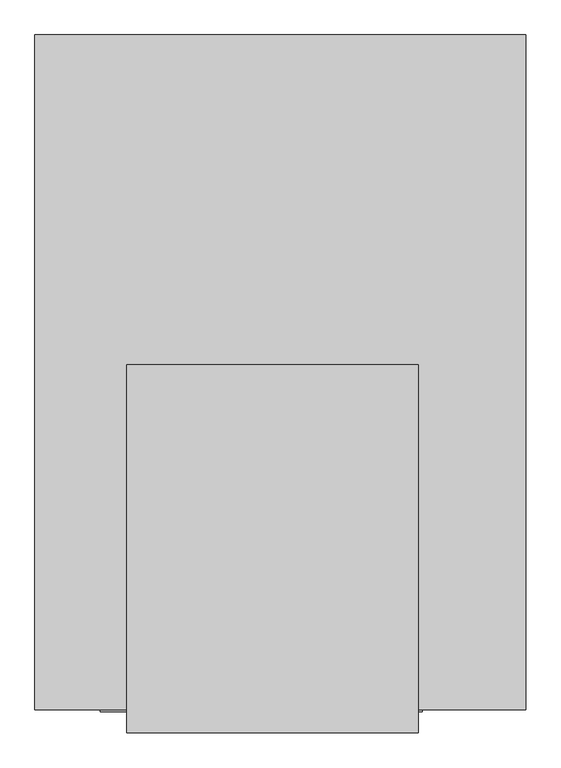
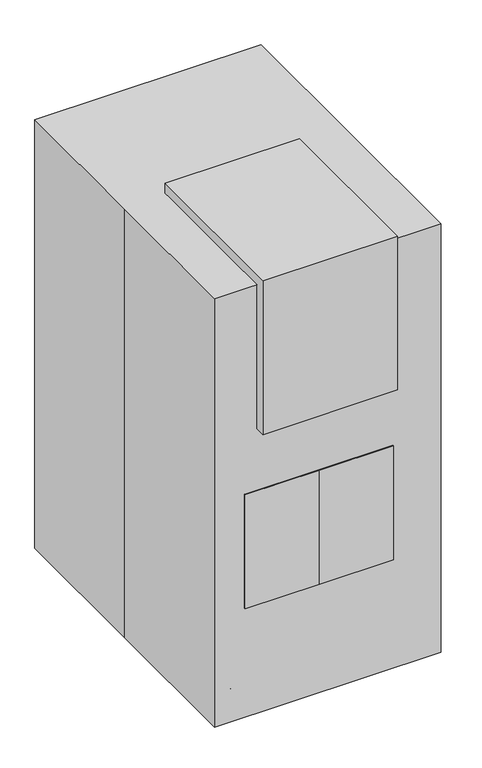
"""IFC4 building model written with IfcOpenShell, lengths in millimetres: proxy geometry, X9500 - System, Uptake, Thyroid, Mobile : X9500 - System, Uptake, Thyroid, Mobile."""

from ifc_helpers import new_model, si_unit, point, frame, frame_2d, origin, origin_with_axes, place, context, project, spatial, polyline, circle_curve, trimmed, segment, composite_curve, outline, extrude, faceted_brep, source, transform, mapped, element, save


def specialty_equipment_a1d769d3(model_context):
    return source(origin(), model_context, "Body", "SolidModel", [
        faceted_brep([(222.25, -92.075, 768.5274151), (-208.9546875, -92.075, 768.5274151), (-208.9546875, -307.975, 768.5274151), (222.25, -307.975, 768.5274151), (222.25, -523.875, 412.9274151), (-208.9546875, -523.875, 412.9274151), (-208.9546875, -92.075, 412.9274151), (222.25, -92.075, 412.9274151), (222.25, -307.975, 735.7348675), (222.25, -523.875, 735.7348675), (222.25, -523.875, 590.7274151), (222.25, -307.975, 590.7274151), (222.25, -307.975, 495.1924677), (222.25, -523.875, 533.6276131), (-208.9546875, -523.875, 533.6276131), (163.7431114, -523.875, 735.7348675), (163.7431114, -523.875, 666.9274151), (-161.3296875, -523.875, 666.9274151), (-161.3296875, -523.875, 735.7348675), (-208.9546875, -523.875, 735.7348675), (-208.9546875, -523.875, 666.9274151), (-285.75, -523.875, 666.9274151), (-285.75, -523.875, 590.7274151), (-285.75, -92.075, 666.9274151), (-285.75, -92.075, 590.7274151), (-208.9546875, -92.075, 590.7274151), (-208.9546875, -92.075, 666.9274151), (163.7431114, -307.975, 735.7348675), (-161.3296875, -307.975, 735.7348675), (-208.9546875, -307.975, 735.7348675), (-161.3296875, -307.975, 666.9274151), (163.7431114, -307.975, 666.9274151), (-208.9546875, -307.975, 590.7274151), (-208.9546875, -307.975, 495.1924677)], [[[0, 1, 2, 3]], [[4, 5, 6, 7]], [[7, 0, 3, 8, 9, 10, 11, 12, 13, 4]], [[13, 14, 5, 4]], [[15, 16, 17, 18, 19, 20, 21, 22, 10, 9]], [[23, 24, 22, 21]], [[7, 6, 25, 24, 23, 26, 1, 0]], [[8, 27, 15, 9]], [[28, 29, 19, 18]], [[3, 2, 29, 28, 30, 31, 27, 8]], [[30, 28, 18, 17]], [[30, 17, 16, 31]], [[16, 15, 27, 31]], [[26, 23, 21, 20]], [[20, 19, 29, 2, 1, 26]], [[10, 22, 24, 25, 32, 11]], [[12, 33, 14, 13]], [[11, 32, 33, 12]], [[25, 6, 5, 14, 33, 32]]]),
        extrude(outline(polyline([(234.95, -561.975), (-31.75, -561.975), (-298.45, -561.975), (-298.45, -53.975), (234.95, -53.975), (234.95, -561.975)])), frame((0.0, 0.0, 412.9274151), z_axis=(0.0, 0.0, 1.0), x_axis=(1.0, 0.0, 0.0)), (0.0, 0.0, 1.0), 431.8),
        faceted_brep([(-145.9656905, -533.4, 1511.3), (-95.3343095, -533.4, 1511.3), (-95.3343095, -50.8, 1511.3), (-145.9656905, -50.8, 1511.3), (-145.9656905, -533.4, 1231.9), (-145.9656905, -50.8, 1231.9), (-95.3343095, -50.8, 1231.9), (-95.3343095, -533.4, 1231.9), (-95.3343095, -63.5, 1498.6), (-95.3343095, -63.5, 1244.6), (-95.3343095, -520.7, 1244.6), (-95.3343095, -520.7, 1498.6), (-100.1205119, -520.7, 1498.6), (-100.1205119, -63.5, 1498.6), (-100.1205119, -520.7, 1244.6), (-100.1205119, -63.5, 1244.6)], [[[0, 1, 2, 3]], [[4, 5, 6, 7]], [[3, 5, 4, 0]], [[2, 6, 5, 3]], [[1, 7, 6, 2], [8, 9, 10, 11]], [[0, 4, 7, 1]], [[12, 13, 8, 11]], [[14, 10, 9, 15]], [[12, 14, 15, 13]], [[13, 15, 9, 8]], [[11, 10, 14, 12]]]),
        extrude(outline(polyline([(1092.2, 203.2), (1104.9, 50.8), (1079.5, 50.8), (1079.5, 203.2), (1092.2, 203.2)])), frame((0.0, -533.4, 0.0), z_axis=(0.0, 1.0, 0.0), x_axis=(0.0, 0.0, 1.0)), (0.0, 0.0, 1.0), 482.6),
        faceted_brep([(-12.7, -439.3218395, 1104.9), (-228.6, -439.3218395, 1104.9), (-228.6, -439.3218395, 1079.5), (-12.7, -439.3218395, 1079.5), (-228.6, -144.8781605, 1104.9), (-12.7, -144.8781605, 1104.9), (-12.7, -144.8781605, 1079.5), (-228.6, -144.8781605, 1079.5), (-209.4656905, -329.0685686, 1111.25), (-209.4656905, -255.1314314, 1111.25), (-209.4656905, -255.1314314, 1104.9), (-209.4656905, -329.0685686, 1104.9), (-209.4656905, -329.0685686, 1371.6), (-209.4656905, -255.1314314, 1371.6), (-145.9656905, -329.0685686, 1371.6), (-145.9656905, -255.1314314, 1371.6), (-145.9656905, -329.0685686, 1320.8), (-145.9656905, -255.1314314, 1320.8), (-184.0656905, -329.0685686, 1320.8), (-184.0656905, -255.1314314, 1320.8), (-184.0656905, -329.0685686, 1104.9), (-184.0656905, -255.1314314, 1104.9)], [[[0, 1, 2, 3]], [[4, 5, 6, 7]], [[8, 9, 10, 11]], [[12, 13, 9, 8]], [[14, 15, 13, 12]], [[16, 17, 15, 14]], [[18, 19, 17, 16]], [[20, 21, 19, 18]], [[0, 5, 4, 1], [11, 10, 21, 20]], [[3, 6, 5, 0]], [[2, 7, 6, 3]], [[1, 4, 7, 2]], [[20, 18, 16, 14, 12, 8, 11]], [[10, 9, 13, 15, 17, 19, 21]]]),
        extrude(outline(polyline([(-254.0, -596.9), (-254.0, 12.7), (228.6, 12.7), (228.6, -596.9), (-254.0, -596.9)])), frame((0.0, 0.0, 1079.5), z_axis=(0.0, 0.0, 1.0), x_axis=(1.0, 0.0, 0.0)), (0.0, 0.0, 1.0), 584.2),
        extrude(outline(composite_curve([segment(polyline([(119.1380154, 235.2310593), (119.1380154, 381.2810593), (123.8052853, 381.2810593), (123.8052853, 235.359733)]), True, "CONTINUOUS"), segment(trimmed(circle_curve(frame_2d((11.7763715, 229.2430177)), 112.1957741), [point((123.8052853, 235.359733))], [point((77.7346619, 138.4829182))], False, "CARTESIAN"), True, "CONTINUOUS"), segment(polyline([(77.7346619, 138.4829182), (-77.7346619, 138.4829182)]), True, "CONTINUOUS"), segment(trimmed(circle_curve(frame_2d((-11.7763715, 229.2430177)), 112.1957741), [point((-77.7346619, 138.4829182))], [point((-123.8052853, 235.359733))], False, "CARTESIAN"), True, "CONTINUOUS"), segment(polyline([(-123.8052853, 235.359733), (-123.8052853, 381.2810593), (-119.1380154, 381.2810593), (-119.1380154, 235.2310593)]), True, "CONTINUOUS"), segment(trimmed(circle_curve(frame_2d((-11.7763715, 229.2430177)), 107.5285042), [point((-119.1380154, 235.2310593))], [point((-76.2, 143.1501881))], True, "CARTESIAN"), True, "CONTINUOUS"), segment(polyline([(-76.2, 143.1501881), (76.2, 143.1501881)]), True, "CONTINUOUS"), segment(trimmed(circle_curve(frame_2d((11.7763715, 229.2430177)), 107.5285042), [point((76.2, 143.1501881))], [point((119.1380154, 235.2310593))], True, "CARTESIAN"), True, "CONTINUOUS")], self_intersect=False)), frame((0.0, 0.0, 1016.0), z_axis=(0.0, 0.0, 1.0), x_axis=(1.0, 0.0, 0.0)), (0.0, 0.0, 1.0), 19.05),
        extrude(outline(polyline([(0.0, 271.5253368), (238.2760308, 271.5253368), (238.2760308, 0.0), (0.0, 0.0), (0.0, 271.5253368)])), frame((119.1380154, 525.6105842, 1054.6277039), z_axis=(0.0, -0.3583679495452942, 0.9335804264972041), x_axis=(-1.0, 0.0, 0.0)), (0.0, 0.0, 1.0), 50.8),
        extrude(outline(polyline([(50.8, 36.8829182), (-50.8, 36.8829182), (-50.8, 138.4829182), (50.8, 138.4829182), (50.8, 36.8829182)])), frame((0.0, 0.0, 1004.2876576), z_axis=(0.0, 0.0, 1.0), x_axis=(1.0, 0.0, 0.0)), (0.0, 0.0, 1.0), 50.8),
        extrude(outline(polyline([(203.2, -547.3170818), (-209.55, -547.3170818), (-209.55, -39.3170818), (203.2, -39.3170818), (203.2, -547.3170818)])), frame((0.0, 0.0, 374.65), z_axis=(0.0, 0.0, 1.0), x_axis=(1.0, 0.0, 0.0)), (0.0, 0.0, 1.0), 38.1),
        extrude(outline(polyline([(-39.3170818, 1041.4), (-39.3170818, 812.8), (-191.7170818, 812.8), (-521.9170818, 1016.0), (-521.9170818, 1041.4), (-39.3170818, 1041.4)])), frame((190.5, 0.0, 0.0), z_axis=(1.0, 0.0, 0.0), x_axis=(0.0, 1.0, 0.0)), (0.0, 0.0, 1.0), 38.1),
        extrude(outline(polyline([(-39.3170818, 1041.4), (-39.3170818, 812.8), (-191.7170818, 812.8), (-521.9170818, 1016.0), (-521.9170818, 1041.4), (-39.3170818, 1041.4)])), frame((-228.6, 0.0, 0.0), z_axis=(1.0, 0.0, 0.0), x_axis=(0.0, 1.0, 0.0)), (0.0, 0.0, 1.0), 38.1),
        extrude(outline(polyline([(247.65, -547.3170818), (-253.5329849, -547.3170818), (-253.5329849, -39.3170818), (247.65, -39.3170818), (247.65, -547.3170818)])), frame((0.0, 0.0, 1041.4), z_axis=(0.0, 0.0, 1.0), x_axis=(1.0, 0.0, 0.0)), (0.0, 0.0, 1.0), 38.1),
        extrude(outline(polyline([(-209.55, -39.3170818), (-209.55, -83.7670818), (-304.8, -83.7670818), (-304.8, 83.7670818), (-209.55, 83.7670818), (-209.55, 36.8829182), (-254.0, 36.8829182), (-254.0, -1.2170818), (-254.0, -39.3170818), (-209.55, -39.3170818)])), frame((0.0, 0.0, 266.7), z_axis=(0.0, 0.0, 1.0), x_axis=(1.0, 0.0, 0.0)), (0.0, 0.0, 1.0), 342.9),
        extrude(outline(polyline([(203.2, -39.3170818), (247.65, -39.3170818), (247.65, -1.2170818), (247.65, 36.8829182), (203.2, 36.8829182), (203.2, 83.7670818), (298.45, 83.7670818), (298.45, -83.7670818), (203.2, -83.7670818), (203.2, -39.3170818)])), frame((0.0, 0.0, 266.7), z_axis=(0.0, 0.0, 1.0), x_axis=(1.0, 0.0, 0.0)), (0.0, 0.0, 1.0), 342.9),
        extrude(outline(polyline([(247.65, -39.3170818), (-253.5329849, -39.3170818), (-253.5329849, 36.8829182), (247.65, 36.8829182), (247.65, -39.3170818)])), frame((0.0, 0.0, 266.7), z_axis=(0.0, 0.0, 1.0), x_axis=(1.0, 0.0, 0.0)), (0.0, 0.0, 1.0), 1248.8024583),
        extrude(outline(polyline([(349.25, -121.8929078), (-355.1329849, -121.8929078), (-355.1329849, 133.5826903), (349.25, 133.5826903), (349.25, -121.8929078)])), frame((0.0, 0.0, 165.1), z_axis=(0.0, 0.0, 1.0), x_axis=(1.0, 0.0, 0.0)), (0.0, 0.0, 1.0), 101.6),
        extrude(outline(composite_curve([segment(trimmed(circle_curve(frame_2d((-306.4724956, 409.1524744)), 16.9333333), [point((-323.405829, 409.1524744))], [point((-289.5391623, 409.1524744))], False, "CARTESIAN"), True, "CONTINUOUS"), segment(trimmed(circle_curve(frame_2d((-306.4724956, 409.1524744)), 16.9333333), [point((-289.5391623, 409.1524744))], [point((-323.405829, 409.1524744))], False, "CARTESIAN"), True, "CONTINUOUS")], self_intersect=False)), frame((0.0, 0.0, 84.8149176), z_axis=(0.0, 0.0, 1.0), x_axis=(1.0, 0.0, 0.0)), (0.0, 0.0, 1.0), 42.1850824),
        extrude(outline(composite_curve([segment(trimmed(circle_curve(frame_2d((297.8141923, 409.1524744)), 16.9333333), [point((314.7475256, 409.1524744))], [point((280.880859, 409.1524744))], False, "CARTESIAN"), True, "CONTINUOUS"), segment(trimmed(circle_curve(frame_2d((297.8141923, 409.1524744)), 16.9333333), [point((280.880859, 409.1524744))], [point((314.7475256, 409.1524744))], False, "CARTESIAN"), True, "CONTINUOUS")], self_intersect=False)), frame((0.0, 0.0, 84.8149176), z_axis=(0.0, 0.0, 1.0), x_axis=(1.0, 0.0, 0.0)), (0.0, 0.0, 1.0), 42.1850824),
        extrude(outline(composite_curve([segment(trimmed(circle_curve(frame_2d((392.219141, 50.8)), 50.8), [point((443.019141, 50.8))], [point((341.419141, 50.8))], False, "CARTESIAN"), True, "CONTINUOUS"), segment(trimmed(circle_curve(frame_2d((392.219141, 50.8)), 50.8), [point((341.419141, 50.8))], [point((443.019141, 50.8))], False, "CARTESIAN"), True, "CONTINUOUS")], self_intersect=False)), frame((261.830859, 0.0, 0.0), z_axis=(1.0, 0.0, 0.0), x_axis=(0.0, 1.0, 0.0)), (0.0, 0.0, 1.0), 19.05),
        extrude(outline(composite_curve([segment(trimmed(circle_curve(frame_2d((392.219141, 50.8)), 50.8), [point((443.019141, 50.8))], [point((341.419141, 50.8))], False, "CARTESIAN"), True, "CONTINUOUS"), segment(trimmed(circle_curve(frame_2d((392.219141, 50.8)), 50.8), [point((341.419141, 50.8))], [point((443.019141, 50.8))], False, "CARTESIAN"), True, "CONTINUOUS")], self_intersect=False)), frame((318.980859, 0.0, 0.0), z_axis=(1.0, 0.0, 0.0), x_axis=(0.0, 1.0, 0.0)), (0.0, 0.0, 1.0), 19.05),
        extrude(outline(composite_curve([segment(trimmed(circle_curve(frame_2d((392.219141, 50.8)), 33.8666667), [point((358.3524744, 50.8))], [point((426.0858077, 50.8))], False, "CARTESIAN"), True, "CONTINUOUS"), segment(trimmed(circle_curve(frame_2d((392.219141, 50.8)), 33.8666667), [point((426.0858077, 50.8))], [point((358.3524744, 50.8))], False, "CARTESIAN"), True, "CONTINUOUS")], self_intersect=False)), frame((280.880859, 0.0, 0.0), z_axis=(1.0, 0.0, 0.0), x_axis=(0.0, 1.0, 0.0)), (0.0, 0.0, 1.0), 38.1),
        extrude(outline(composite_curve([segment(trimmed(circle_curve(frame_2d((392.219141, 50.8)), 50.8), [point((443.019141, 50.8))], [point((341.419141, 50.8))], False, "CARTESIAN"), True, "CONTINUOUS"), segment(trimmed(circle_curve(frame_2d((392.219141, 50.8)), 50.8), [point((341.419141, 50.8))], [point((443.019141, 50.8))], False, "CARTESIAN"), True, "CONTINUOUS")], self_intersect=False)), frame((-287.230859, 0.0, 0.0), z_axis=(1.0, 0.0, 0.0), x_axis=(0.0, 1.0, 0.0)), (0.0, 0.0, 1.0), 19.05),
        extrude(outline(composite_curve([segment(trimmed(circle_curve(frame_2d((392.219141, 50.8)), 50.8), [point((443.019141, 50.8))], [point((341.419141, 50.8))], False, "CARTESIAN"), True, "CONTINUOUS"), segment(trimmed(circle_curve(frame_2d((392.219141, 50.8)), 50.8), [point((341.419141, 50.8))], [point((443.019141, 50.8))], False, "CARTESIAN"), True, "CONTINUOUS")], self_intersect=False)), frame((-344.380859, 0.0, 0.0), z_axis=(1.0, 0.0, 0.0), x_axis=(0.0, 1.0, 0.0)), (0.0, 0.0, 1.0), 19.05),
        extrude(outline(composite_curve([segment(trimmed(circle_curve(frame_2d((392.219141, 50.8)), 33.8666667), [point((358.3524744, 50.8))], [point((426.0858077, 50.8))], False, "CARTESIAN"), True, "CONTINUOUS"), segment(trimmed(circle_curve(frame_2d((392.219141, 50.8)), 33.8666667), [point((426.0858077, 50.8))], [point((358.3524744, 50.8))], False, "CARTESIAN"), True, "CONTINUOUS")], self_intersect=False)), frame((-325.330859, 0.0, 0.0), z_axis=(1.0, 0.0, 0.0), x_axis=(0.0, 1.0, 0.0)), (0.0, 0.0, 1.0), 38.1),
        extrude(outline(polyline([(-253.5329849, -438.15), (-355.1329849, -438.15), (-355.1329849, 457.2), (-253.5329849, 457.2), (-253.5329849, -438.15)])), frame((0.0, 0.0, 127.0), z_axis=(0.0, 0.0, 1.0), x_axis=(1.0, 0.0, 0.0)), (0.0, 0.0, 1.0), 38.1),
        extrude(outline(polyline([(349.25, -438.15), (247.65, -438.15), (247.65, 457.2), (349.25, 457.2), (349.25, -438.15)])), frame((0.0, 0.0, 127.0), z_axis=(0.0, 0.0, 1.0), x_axis=(1.0, 0.0, 0.0)), (0.0, 0.0, 1.0), 38.1),
        extrude(outline(composite_curve([segment(trimmed(circle_curve(frame_2d((-306.4724956, -371.8975256)), 16.9333333), [point((-323.405829, -371.8975256))], [point((-289.5391623, -371.8975256))], False, "CARTESIAN"), True, "CONTINUOUS"), segment(trimmed(circle_curve(frame_2d((-306.4724956, -371.8975256)), 16.9333333), [point((-289.5391623, -371.8975256))], [point((-323.405829, -371.8975256))], False, "CARTESIAN"), True, "CONTINUOUS")], self_intersect=False)), frame((0.0, 0.0, 84.8149176), z_axis=(0.0, 0.0, 1.0), x_axis=(1.0, 0.0, 0.0)), (0.0, 0.0, 1.0), 42.1850824),
        extrude(outline(composite_curve([segment(trimmed(circle_curve(frame_2d((297.8141923, -371.8975256)), 16.9333333), [point((314.7475256, -371.8975256))], [point((280.880859, -371.8975256))], False, "CARTESIAN"), True, "CONTINUOUS"), segment(trimmed(circle_curve(frame_2d((297.8141923, -371.8975256)), 16.9333333), [point((280.880859, -371.8975256))], [point((314.7475256, -371.8975256))], False, "CARTESIAN"), True, "CONTINUOUS")], self_intersect=False)), frame((0.0, 0.0, 84.8149176), z_axis=(0.0, 0.0, 1.0), x_axis=(1.0, 0.0, 0.0)), (0.0, 0.0, 1.0), 42.1850824),
        extrude(outline(composite_curve([segment(trimmed(circle_curve(frame_2d((-388.830859, 50.8)), 50.8), [point((-338.030859, 50.8))], [point((-439.630859, 50.8))], False, "CARTESIAN"), True, "CONTINUOUS"), segment(trimmed(circle_curve(frame_2d((-388.830859, 50.8)), 50.8), [point((-439.630859, 50.8))], [point((-338.030859, 50.8))], False, "CARTESIAN"), True, "CONTINUOUS")], self_intersect=False)), frame((261.830859, 0.0, 0.0), z_axis=(1.0, 0.0, 0.0), x_axis=(0.0, 1.0, 0.0)), (0.0, 0.0, 1.0), 19.05),
        extrude(outline(composite_curve([segment(trimmed(circle_curve(frame_2d((-388.830859, 50.8)), 50.8), [point((-338.030859, 50.8))], [point((-439.630859, 50.8))], False, "CARTESIAN"), True, "CONTINUOUS"), segment(trimmed(circle_curve(frame_2d((-388.830859, 50.8)), 50.8), [point((-439.630859, 50.8))], [point((-338.030859, 50.8))], False, "CARTESIAN"), True, "CONTINUOUS")], self_intersect=False)), frame((318.980859, 0.0, 0.0), z_axis=(1.0, 0.0, 0.0), x_axis=(0.0, 1.0, 0.0)), (0.0, 0.0, 1.0), 19.05),
        extrude(outline(composite_curve([segment(trimmed(circle_curve(frame_2d((-388.830859, 50.8)), 33.8666667), [point((-422.6975256, 50.8))], [point((-354.9641923, 50.8))], False, "CARTESIAN"), True, "CONTINUOUS"), segment(trimmed(circle_curve(frame_2d((-388.830859, 50.8)), 33.8666667), [point((-354.9641923, 50.8))], [point((-422.6975256, 50.8))], False, "CARTESIAN"), True, "CONTINUOUS")], self_intersect=False)), frame((280.880859, 0.0, 0.0), z_axis=(1.0, 0.0, 0.0), x_axis=(0.0, 1.0, 0.0)), (0.0, 0.0, 1.0), 38.1),
        extrude(outline(composite_curve([segment(trimmed(circle_curve(frame_2d((-388.830859, 50.8)), 50.8), [point((-338.030859, 50.8))], [point((-439.630859, 50.8))], False, "CARTESIAN"), True, "CONTINUOUS"), segment(trimmed(circle_curve(frame_2d((-388.830859, 50.8)), 50.8), [point((-439.630859, 50.8))], [point((-338.030859, 50.8))], False, "CARTESIAN"), True, "CONTINUOUS")], self_intersect=False)), frame((-287.230859, 0.0, 0.0), z_axis=(1.0, 0.0, 0.0), x_axis=(0.0, 1.0, 0.0)), (0.0, 0.0, 1.0), 19.05),
        extrude(outline(composite_curve([segment(trimmed(circle_curve(frame_2d((-388.830859, 50.8)), 50.8), [point((-338.030859, 50.8))], [point((-439.630859, 50.8))], False, "CARTESIAN"), True, "CONTINUOUS"), segment(trimmed(circle_curve(frame_2d((-388.830859, 50.8)), 50.8), [point((-439.630859, 50.8))], [point((-338.030859, 50.8))], False, "CARTESIAN"), True, "CONTINUOUS")], self_intersect=False)), frame((-344.380859, 0.0, 0.0), z_axis=(1.0, 0.0, 0.0), x_axis=(0.0, 1.0, 0.0)), (0.0, 0.0, 1.0), 19.05),
        extrude(outline(composite_curve([segment(trimmed(circle_curve(frame_2d((-388.830859, 50.8)), 33.8666667), [point((-422.6975256, 50.8))], [point((-354.9641923, 50.8))], False, "CARTESIAN"), True, "CONTINUOUS"), segment(trimmed(circle_curve(frame_2d((-388.830859, 50.8)), 33.8666667), [point((-354.9641923, 50.8))], [point((-422.6975256, 50.8))], False, "CARTESIAN"), True, "CONTINUOUS")], self_intersect=False)), frame((-325.330859, 0.0, 0.0), z_axis=(1.0, 0.0, 0.0), x_axis=(0.0, 1.0, 0.0)), (0.0, 0.0, 1.0), 38.1),
        extrude(outline(polyline([(-406.4, -558.8), (-406.4, 0.0), (-406.4, 558.8), (406.4, 558.8), (406.4, -558.8), (-406.4, -558.8)])), origin_with_axes(), (0.0, 0.0, 1.0), 1625.6),
    ])


if __name__ == "__main__":
    model = new_model("IFC4")
    model_context = context("Model", 3, world=origin())
    ifc_project = project(units=[si_unit("LENGTHUNIT", "METRE", prefix="MILLI")], contexts=[model_context])
    site = spatial("IfcSite", under=ifc_project)
    building = spatial("IfcBuilding", under=site)
    placement = place(None, origin())
    specialty_equipment_shape = specialty_equipment_a1d769d3(model_context)
    element("IfcBuildingElementProxy", 1, Name="X9500 - System, Uptake, Thyroid, Mobile : X9500 - System, Uptake, Thyroid, Mobile", ObjectType="X9500 - System, Uptake, Thyroid, Mobile : X9500 - System, Uptake, Thyroid, Mobile", at=placement, inside=building, context=model_context, shape_type="MappedRepresentation", body=[
        mapped(specialty_equipment_shape, transform((0.0, 0.0, 0.0), x_axis=(1.0, 0.0, 0.0), y_axis=(0.0, 1.0, 0.0), z_axis=(0.0, 0.0, 1.0))),
    ])
    save(model, "model.ifc")

# Revit data of these elements
# Project information
#   Sheets - Total = "5"
#   Project Issue Date = "Issue Date"
#   Project Status = "Project Status"
#   Client Name = "Owner"
#   Project Address = "Enter address here"
#   Project Name = "Project Name"
#   Project Number = "Project Number"
#   Publication Date = "30-Jan-15"
# Type "X9500 - System, Uptake, Thyroid, Mobile : X9500 - System, Uptake, Thyroid, Mobile"
#   Watts2 = "0"
#   Watts1 = "720"
#   Unit_Issue = "EA"
#   UTIL_6_Misc = "-"
#   UTIL_5_NonMedGas = "-"
#   UTIL_4_MiscGas = "-"
#   UTIL_3_MedGas = "-"
#   UTIL_2_Elec = "B"
#   UTIL_1_WaterDrain = "-"
#   Nomenclature = "System, Uptake, Thyroid, Mobile"
#   NSN = "6525"
#   Location [instance default] = ""
#   JSN = "X9500"
#   Fund_Source_VA = "-"
#   Fund_Source_Navy = "-"
#   Fund_Source_Army = "-"
#   Fund_Source_AF = "-"
#   ELEC_Volts2 = "0"
#   ELEC_Volts1 = "120"
#   ELEC_Phase2 = "0"
#   ELEC_Phase1 = "1"
#   ELEC_HertzSwitch = "-1"
#   ELEC_HertzDependent = "0"
#   ELEC_Hertz = "50/60"
#   ELEC_Amps2 = "0"
#   ELEC_Amps1 = "6"
#   DetailDescription = "Mobile thyroid uptake system. The characteristics and components include; amplifier tube assembly and base, uptake stand and collimated shield. This is a mobile unit with arm medical stand, 2 inch probe with I.A.E.A. flat field collimator and thyroid positioner, neck phantom, and analyzer/scaler/timer with automatic background subtract and automatic % readout."
#   CAT_VA = "C"
#   CAT_Navy = "C"
#   CAT_IHS = "-"
#   CAT_Army = "C"
#   CAT_AF = "C"
#   BTUperhour = "0"
#   radius = 0' - 2"
#   calc 2 = 0' - 0.66667"
#   calc 1 = 0' - 1.33333"
#   Weight_IP = 450
#   DIM_Width_IP = 2' - 8"
#   DIM_Height_IP = 5' - 4"
#   DIM_Depth_IP = 3' - 8"
#   top [instance default] = none
#   finish [instance default] = none
# Element 1 (IfcBuildingElementProxy, "X9500 - System, Uptake, Thyroid, Mobile : X9500 - System, Uptake, Thyroid, Mobile")
#   Materials on its faces: "EquipSpace"
# Materials
#   "EquipSpace": class "Unassigned", colour RGB 221 217 195, transparency 0.5
